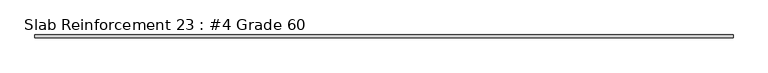
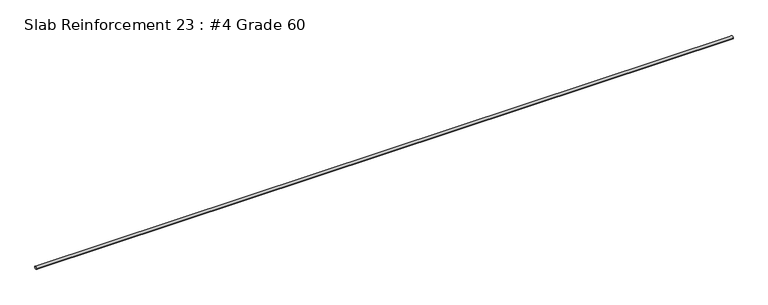
"""IFC4 building model written with IfcOpenShell, lengths in millimetres: proxy geometry, Slab Reinforcement 23 : #4 Grade 60."""

from ifc_helpers import new_model, si_unit, point, frame, frame_2d, origin, place, context, project, spatial, circle_curve, trimmed, segment, composite_curve, outline, extrude, source, transform, mapped, element, save


def slab_reinforcement_23_4_grade_60_863f9fcf(model_context):
    return source(origin(), model_context, "Body", "SweptSolid", [
        extrude(outline(composite_curve([segment(trimmed(circle_curve(frame_2d((-534045.8663841, -82.55)), 6.35), [point((-534052.2163841, -82.55))], [point((-534039.5163841, -82.55))], False, "CARTESIAN"), True, "CONTINUOUS"), segment(trimmed(circle_curve(frame_2d((-534045.8663841, -82.55)), 6.35), [point((-534039.5163841, -82.55))], [point((-534052.2163841, -82.55))], False, "CARTESIAN"), True, "CONTINUOUS")], self_intersect=False)), frame((587369.3484865, 0.0, 0.0), z_axis=(1.0, 0.0, 0.0), x_axis=(0.0, 1.0, 0.0)), (0.0, 0.0, 1.0), 2946.4),
    ])


if __name__ == "__main__":
    model = new_model("IFC4")
    model_context = context("Model", 3, world=origin())
    ifc_project = project(units=[si_unit("LENGTHUNIT", "METRE", prefix="MILLI")], contexts=[model_context])
    site = spatial("IfcSite", under=ifc_project)
    building = spatial("IfcBuilding", under=site)
    placement = place(None, origin())
    slab_reinforcement_23_4_grade_60_shape = slab_reinforcement_23_4_grade_60_863f9fcf(model_context)
    element("IfcBuildingElementProxy", 1, Name="Slab Reinforcement 23 : #4 Grade 60", ObjectType="Slab Reinforcement 23 : #4 Grade 60", at=placement, inside=building, context=model_context, shape_type="MappedRepresentation", body=[
        mapped(slab_reinforcement_23_4_grade_60_shape, transform((0.0, 0.0, 0.0), x_axis=(1.0, 0.0, 0.0), y_axis=(0.0, 1.0, 0.0), z_axis=(0.0, 0.0, 1.0))),
    ])
    save(model, "model.ifc")

# Revit data of these elements
# Element 1 (IfcBuildingElementProxy, "Slab Reinforcement 23 : #4 Grade 60")
#   Materials on its faces: "#4 GR. 60 REINF. @ 16\" O.C. EW."
# Materials
#   "#4 GR. 60 REINF. @ 16\" O.C. EW.": class "Generic", colour RGB 84 83 81, transparency 0, Cost = 0
